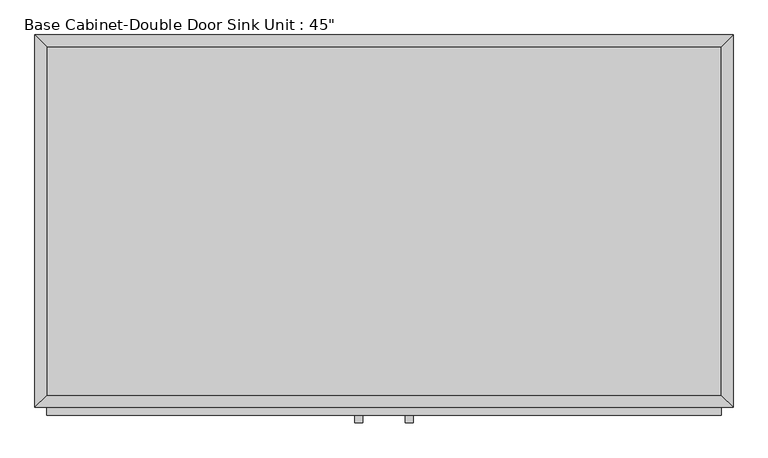
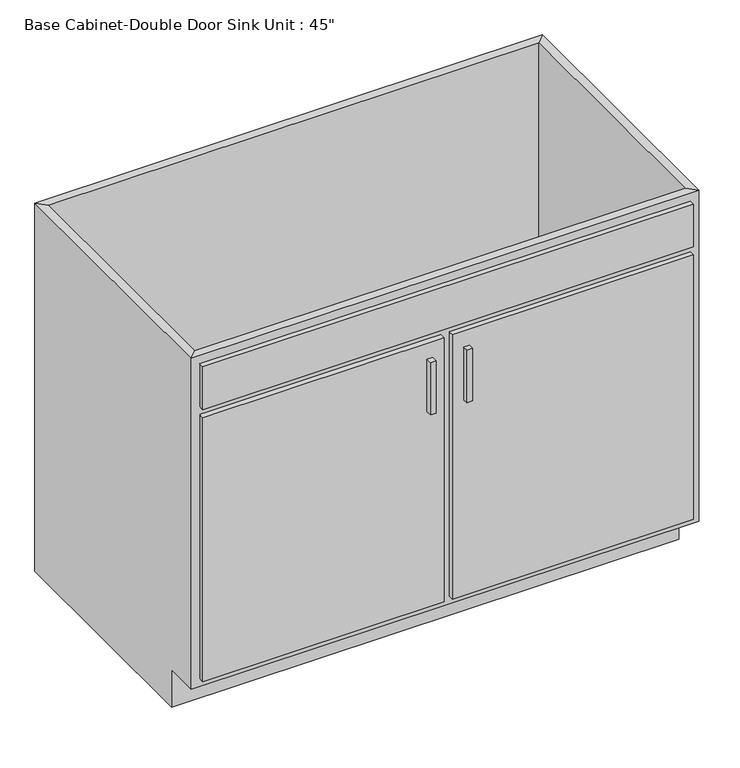
"""IFC4 building model written with IfcOpenShell, lengths in millimetres: furniture geometry."""

import ifcopenshell
import ifcopenshell.guid

model = None  # the IFC model being written
_history = None  # IfcOwnerHistory: only IFC2X3 demands one
_inside = {}  # id of a spatial element -> (the spatial element, [elements in it])
_under = {}  # id of a project, library or spatial element -> (it, [spatial elements below it])
_declared = {}  # id of a project -> (the project, [libraries it declares])
_typed = {}  # id of a type object -> (the type object, [elements of that type])
_made_of = {}  # id of a material, layer set ... -> (it, [elements and type objects made of it])


def new_model(schema):
    """Start an empty IFC model of exactly this schema.

    Asked for "IFC4X3", IfcOpenShell would pick the latest addendum, in which some entities
    have other attributes; the version numbers below select the first issue.
    IFC2X3 requires an IfcOwnerHistory on every rooted entity: one is made here for all.
    """
    global model, _history
    if schema == "IFC4X3":
        model = ifcopenshell.file(schema_version=(4, 3, 0, 0))
    else:
        model = ifcopenshell.file(schema=schema)
    _inside.clear()
    _under.clear()
    _declared.clear()
    _typed.clear()
    _made_of.clear()
    _history = None
    if model.schema == "IFC2X3":
        org = make("IfcOrganization", Name="unknown")
        user = make(
            "IfcPersonAndOrganization",
            ThePerson=make("IfcPerson", FamilyName="unknown"),
            TheOrganization=org,
        )
        app = make(
            "IfcApplication",
            ApplicationDeveloper=org,
            Version="unknown",
            ApplicationFullName="unknown",
            ApplicationIdentifier="unknown",
        )
        _history = make(
            "IfcOwnerHistory",
            OwningUser=user,
            OwningApplication=app,
            ChangeAction="ADDED",
            CreationDate=0,
        )
    return model


def make(cls, **values):
    """One entity of the class cls with the attributes given. An attribute that is None is left unset."""
    return model.create_entity(
        cls, **{name: value for name, value in values.items() if value is not None}
    )


def rooted(cls, **values):
    """An entity with a GlobalId (a new one), such as an element, a storey or a relation."""
    return make(cls, GlobalId=ifcopenshell.guid.new(), OwnerHistory=_history, **values)


def si_unit(unit_type, name, prefix=None):
    """IfcSIUnit, for example si_unit("LENGTHUNIT", "METRE", prefix="MILLI")."""
    return make("IfcSIUnit", UnitType=unit_type, Prefix=prefix, Name=name)


def assignment(units):
    """IfcUnitAssignment: the units of a project."""
    return None if units is None else make("IfcUnitAssignment", Units=units)


def point(xyz):
    """IfcCartesianPoint."""
    return None if xyz is None else make("IfcCartesianPoint", Coordinates=xyz)


def direction(xyz):
    """IfcDirection."""
    return None if xyz is None else make("IfcDirection", DirectionRatios=xyz)


def frame(location, z_axis=None, x_axis=None):
    """IfcAxis2Placement3D, a coordinate frame: its origin and axes. An axis left out is left unset."""
    return make(
        "IfcAxis2Placement3D",
        Location=point(location),
        Axis=direction(z_axis),
        RefDirection=direction(x_axis),
    )


def origin():
    """The frame at (0, 0, 0) with its axes left unset."""
    return frame((0.0, 0.0, 0.0))


def place(relative_to, where):
    """IfcLocalPlacement: puts the frame where relative to a parent placement (None: the world)."""
    return make(
        "IfcLocalPlacement", PlacementRelTo=relative_to, RelativePlacement=where
    )


def context(
    kind, dimensions, precision=None, world=None, true_north=None, identifier=None
):
    """IfcGeometricRepresentationContext, for example the 3D "Model" context."""
    return make(
        "IfcGeometricRepresentationContext",
        ContextIdentifier=identifier,
        ContextType=kind,
        CoordinateSpaceDimension=dimensions,
        Precision=precision,
        WorldCoordinateSystem=world,
        TrueNorth=true_north,
    )


def project(units=None, contexts=None):
    """IfcProject with its units and contexts."""
    return rooted(
        "IfcProject",
        Name="project",
        RepresentationContexts=contexts,
        UnitsInContext=assignment(units),
    )


def spatial(cls, under=None, at=None, **own):
    """A site, building, storey or space (cls), placed at a placement, below another one or the project."""
    s = rooted(cls, ObjectPlacement=at, **own)
    if under is not None:
        _under.setdefault(under.id(), (under, []))[1].append(s)
    return s


def polyline(points):
    """IfcPolyline through the points."""
    return make("IfcPolyline", Points=[point(p) for p in points])


def outline(outer, holes=None, kind="AREA"):
    """IfcArbitraryClosedProfileDef: a profile drawn as a closed curve; with holes, ...WithVoids."""
    if holes is None:
        return make("IfcArbitraryClosedProfileDef", ProfileType=kind, OuterCurve=outer)
    return make(
        "IfcArbitraryProfileDefWithVoids",
        ProfileType=kind,
        OuterCurve=outer,
        InnerCurves=holes,
    )


def extrude(swept, where, along, depth):
    """IfcExtrudedAreaSolid: the profile swept, set in the frame where, extruded along a direction by depth."""
    return make(
        "IfcExtrudedAreaSolid",
        SweptArea=swept,
        Position=where,
        ExtrudedDirection=direction(along),
        Depth=depth,
    )


def faces_of(points, faces, orient=None, outer=None):
    """IfcFace entities. A face is a list of loops; a loop is a list of indices into points, from 0.

    orient and outer hold one flag for each loop. By default every Orientation is true, the
    first loop of a face is its IfcFaceOuterBound and the others are IfcFaceBound.
    """
    made = []
    for i, loops in enumerate(faces):
        bounds = []
        for j, loop in enumerate(loops):
            is_outer = j == 0 if outer is None else outer[i][j]
            bounds.append(
                make(
                    "IfcFaceOuterBound" if is_outer else "IfcFaceBound",
                    Bound=make("IfcPolyLoop", Polygon=[points[k] for k in loop]),
                    Orientation=True if orient is None else orient[i][j],
                )
            )
        made.append(make("IfcFace", Bounds=bounds))
    return made


def faceted_brep(points, faces, orient=None, outer=None, voids=None):
    """IfcFacetedBrep: a solid bounded by flat faces; with voids (closed shells), ...WithVoids."""
    shared = [point(p) for p in points]
    hull = make("IfcClosedShell", CfsFaces=faces_of(shared, faces, orient, outer))
    if voids is None:
        return make("IfcFacetedBrep", Outer=hull)
    return make(
        "IfcFacetedBrepWithVoids",
        Outer=hull,
        Voids=[
            make(cls, CfsFaces=faces_of(shared, fs, o, b)) for cls, fs, o, b in voids
        ],
    )


def shape(context_of_items, identifier, shape_type, items):
    """IfcShapeRepresentation: the items that make up one representation, for example the "Body"."""
    return make(
        "IfcShapeRepresentation",
        ContextOfItems=context_of_items,
        RepresentationIdentifier=identifier,
        RepresentationType=shape_type,
        Items=items,
    )


def source(mapping_origin, context_of_items, identifier, shape_type, items):
    """IfcRepresentationMap: a shape defined once, which mapped items show again and again."""
    return make(
        "IfcRepresentationMap",
        MappingOrigin=mapping_origin,
        MappedRepresentation=shape(context_of_items, identifier, shape_type, items),
    )


def transform(
    local_origin,
    x_axis=None,
    y_axis=None,
    z_axis=None,
    scale=None,
    scale2=None,
    scale3=None,
    uniform=True,
):
    """IfcCartesianTransformationOperator3D, or its non-uniform kind. x_axis, y_axis, z_axis: its Axis1, 2, 3."""
    if uniform:
        return make(
            "IfcCartesianTransformationOperator3D",
            Axis1=direction(x_axis),
            Axis2=direction(y_axis),
            LocalOrigin=point(local_origin),
            Scale=scale,
            Axis3=direction(z_axis),
        )
    return make(
        "IfcCartesianTransformationOperator3DnonUniform",
        Axis1=direction(x_axis),
        Axis2=direction(y_axis),
        LocalOrigin=point(local_origin),
        Scale=scale,
        Axis3=direction(z_axis),
        Scale2=scale2,
        Scale3=scale3,
    )


def mapped(mapping_source, mapping_target):
    """IfcMappedItem: shows the shape of a source again, moved by a transform."""
    return make(
        "IfcMappedItem", MappingSource=mapping_source, MappingTarget=mapping_target
    )


def made_of(thing, what):
    """Note that an element or type object is made of a material, layer set ...; save() writes the relation."""
    if what is not None:
        _made_of.setdefault(what.id(), (what, []))[1].append(thing)
    return thing


def element(
    cls,
    number,
    at=None,
    inside=None,
    cuts=None,
    type_object=None,
    material=None,
    context=None,
    identifier="Body",
    shape_type=None,
    held_by="IfcProductDefinitionShape",
    body=None,
    shapes=None,
    **own,
):
    """One element of the class cls, such as IfcWall. Its Tag is "e" and its number.

    at: its placement. inside: the storey or other place that contains it. cuts: it is an
    opening in that element (IfcRelVoidsElement). A single representation is given by context,
    identifier, shape_type and body (its items); several are given by shapes. held_by: the class
    of the entity that holds the representations. save() writes the other relations.
    """
    e = rooted(cls, Tag="e%d" % number, ObjectPlacement=at, **own)
    if body is not None:
        shapes = [shape(context, identifier, shape_type, body)]
    if shapes is not None:
        e.Representation = make(held_by, Representations=shapes)
    if inside is not None:
        _inside.setdefault(inside.id(), (inside, []))[1].append(e)
    if cuts is not None:
        rooted(
            "IfcRelVoidsElement", RelatingBuildingElement=cuts, RelatedOpeningElement=e
        )
    if type_object is not None:
        _typed.setdefault(type_object.id(), (type_object, []))[1].append(e)
    return made_of(e, material)


def aggregate(whole, parts):
    """IfcRelAggregates: a whole, such as a stair, and the parts it consists of."""
    return rooted("IfcRelAggregates", RelatingObject=whole, RelatedObjects=parts)


def save(model, path):
    """Write the relations noted so far, then the file.

    IfcRelAggregates (storeys below a building ...), IfcRelContainedInSpatialStructure (elements
    in a storey), IfcRelDefinesByType, IfcRelAssociatesMaterial and IfcRelDeclares: one each for
    every whole, place, type object, material and project.
    """
    for whole, parts in _under.values():
        aggregate(whole, parts)
    for where, things in _inside.values():
        rooted(
            "IfcRelContainedInSpatialStructure",
            RelatedElements=things,
            RelatingStructure=where,
        )
    for kind, things in _typed.values():
        rooted("IfcRelDefinesByType", RelatedObjects=things, RelatingType=kind)
    for what, things in _made_of.values():
        rooted("IfcRelAssociatesMaterial", RelatedObjects=things, RelatingMaterial=what)
    for by, libraries in _declared.values():
        rooted("IfcRelDeclares", RelatingContext=by, RelatedDefinitions=libraries)
    model.write(path)


def furniture_6d745834(model_context):
    return source(origin(), model_context, "Body", "SolidModel", [
        faceted_brep([(571.1877049, -590.55, 876.3), (571.1877049, -590.55, 88.9), (-533.7122951, -590.55, 88.9), (-533.7122951, -590.55, 876.3), (-552.7622951, -609.6, 876.3), (590.2377049, -609.6, 876.3), (-552.7622951, -609.6, 88.9), (590.2377049, -609.6, 88.9), (-533.7122951, -533.4, 88.9), (-533.7122951, -19.05, 88.9), (-533.7122951, -19.05, 876.3), (-552.7622951, 0.0, 876.3), (-552.7622951, 0.0, 0.0), (-552.7622951, -533.4, 0.0), (-552.7622951, -533.4, 88.9), (571.1877049, -19.05, 88.9), (571.1877049, -19.05, 876.3), (590.2377049, 0.0, 876.3), (590.2377049, 0.0, 0.0), (571.1877049, -533.4, 88.9), (590.2377049, -533.4, 88.9), (590.2377049, -533.4, 0.0)], [[[0, 1, 2, 3]], [[0, 3, 4, 5]], [[5, 4, 6, 7]], [[2, 1, 7, 6]], [[3, 2, 8, 9, 10]], [[4, 3, 10, 11]], [[6, 4, 11, 12, 13, 14]], [[2, 6, 14, 8]], [[10, 9, 15, 16]], [[11, 10, 16, 17]], [[12, 11, 17, 18]], [[1, 0, 16, 15, 19]], [[0, 5, 17, 16]], [[5, 7, 20, 21, 18, 17]], [[7, 1, 19, 20]], [[8, 19, 15, 9]], [[18, 21, 13, 12]], [[13, 21, 20, 19, 8, 14]]]),
        extrude(outline(polyline([(-16.1872951, -635.0), (-28.8872951, -635.0), (-28.8872951, -622.3), (-16.1872951, -622.3), (-16.1872951, -635.0)])), frame((0.0, 0.0, 573.769895), z_axis=(0.0, 0.0, 1.0), x_axis=(1.0, 0.0, 0.0)), (0.0, 0.0, 1.0), 124.730105),
        extrude(outline(polyline([(66.3627049, -635.0), (53.6627049, -635.0), (53.6627049, -622.3), (66.3627049, -622.3), (66.3627049, -635.0)])), frame((0.0, 0.0, 573.769895), z_axis=(0.0, 0.0, 1.0), x_axis=(1.0, 0.0, 0.0)), (0.0, 0.0, 1.0), 124.730105),
        extrude(outline(polyline([(571.1877049, -19.05), (571.1877049, -590.55), (-533.7122951, -590.55), (-533.7122951, -19.05), (571.1877049, -19.05)])), frame((0.0, 0.0, 88.9), z_axis=(0.0, 0.0, 1.0), x_axis=(1.0, 0.0, 0.0)), (0.0, 0.0, 1.0), 19.05),
        extrude(outline(polyline([(9.2127049, -622.3), (-533.7122951, -622.3), (-533.7122951, -609.6), (9.2127049, -609.6), (9.2127049, -622.3)])), frame((0.0, 0.0, 107.95), z_axis=(0.0, 0.0, 1.0), x_axis=(1.0, 0.0, 0.0)), (0.0, 0.0, 1.0), 628.65),
        extrude(outline(polyline([(571.1877049, -622.3), (28.2627049, -622.3), (28.2627049, -609.6), (571.1877049, -609.6), (571.1877049, -622.3)])), frame((0.0, 0.0, 107.95), z_axis=(0.0, 0.0, 1.0), x_axis=(1.0, 0.0, 0.0)), (0.0, 0.0, 1.0), 628.65),
        extrude(outline(polyline([(571.1877049, -622.3), (-533.7122951, -622.3), (-533.7122951, -609.6), (571.1877049, -609.6), (571.1877049, -622.3)])), frame((0.0, 0.0, 755.65), z_axis=(0.0, 0.0, 1.0), x_axis=(1.0, 0.0, 0.0)), (0.0, 0.0, 1.0), 101.6),
    ])


if __name__ == "__main__":
    model = new_model("IFC4")
    model_context = context("Model", 3, world=origin())
    ifc_project = project(units=[si_unit("LENGTHUNIT", "METRE", prefix="MILLI")], contexts=[model_context])
    site = spatial("IfcSite", under=ifc_project)
    building = spatial("IfcBuilding", under=site)
    placement = place(None, origin())
    furniture_shape = furniture_6d745834(model_context)
    element("IfcFurniture", 1, ObjectType="Base Cabinet-Double Door Sink Unit : 45\"", at=placement, inside=building, context=model_context, shape_type="MappedRepresentation", body=[
        mapped(furniture_shape, transform((0.0, 0.0, 0.0), x_axis=(1.0, 0.0, 0.0), y_axis=(0.0, 1.0, 0.0), z_axis=(0.0, 0.0, 1.0))),
    ])
    save(model, "model.ifc")

# Revit data of these elements
# Type "Base Cabinet-Double Door Sink Unit : 45\""
#   Assembly Code = "C1030410"
#   Depth = 2' - 0"
#   Height = 2' - 10 1/2"
#   Toe Depth = 0' - 3"
#   Toe Height = 0' - 3 1/2"
#   Width = 3' - 9"
#   Cabinet Material = none
#   Door/Drawer Material = none
#   Handle Material = Cabinets - Handles
#   Default Elevation = 0
# Element 1 (IfcFurniture, "Base Cabinet-Double Door Sink Unit : 45\"")
#   Materials on its faces: "Cabinets", "Cabinets - Handles"
# Materials
#   "Cabinets - Handles": class "Metal", colour RGB 57 57 57, transparency 0
#   "Cabinets": class "Miscellaneous", colour RGB 249 249 249, transparency 0
